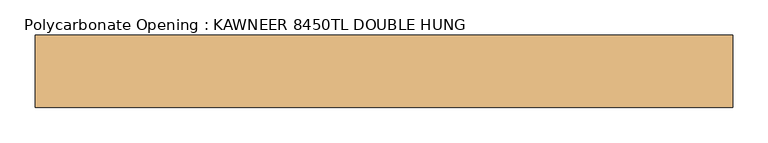
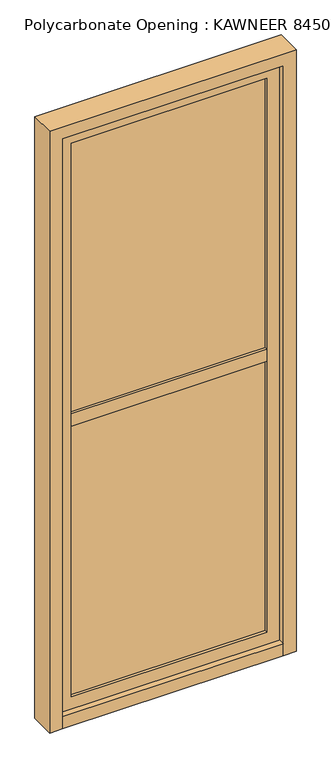
"""IFC4 building model written with IfcOpenShell, lengths in millimetres: door geometry, Polycarbonate Opening : KAWNEER 8450TL DOUBLE HUNG."""

from ifc_helpers import new_model, si_unit, frame, origin, origin_with_axes, place, context, project, spatial, polyline, outline, extrude, source, transform, mapped, element, save


def polycarbonate_opening_kawneer_8450tl_double_hung_37ce2fd3(model_context):
    return source(origin(), model_context, "Body", "SweptSolid", [
        extrude(outline(polyline([(440.1908884, 12.7), (440.1908884, -12.7), (-440.1908884, -12.7), (-440.1908884, 12.7), (440.1908884, 12.7)])), frame((0.0, 0.0, 50.8), z_axis=(0.0, 0.0, 1.0), x_axis=(1.0, 0.0, 0.0)), (0.0, 0.0, 1.0), 2434.1710618),
        extrude(outline(polyline([(2484.9710618, -440.1908884), (0.0, -440.1908884), (0.0, 440.1908884), (2484.9710618, 440.1908884), (2484.9710618, -440.1908884)]), holes=[polyline([(101.6, 389.3908884), (101.6, -389.3908884), (2434.1710618, -389.3908884), (2434.1710618, 389.3908884), (101.6, 389.3908884)])]), frame((0.0, -25.4, 0.0), z_axis=(0.0, 1.0, 0.0), x_axis=(0.0, 0.0, 1.0)), (0.0, 0.0, 1.0), 50.8),
        extrude(outline(polyline([(2535.7710618, 490.9908884), (2535.7710618, -490.9908884), (0.0, -490.9908884), (0.0, -440.1908884), (2484.9710618, -440.1908884), (2484.9710618, 440.1908884), (0.0, 440.1908884), (0.0, 490.9908884), (2535.7710618, 490.9908884)])), frame((0.0, -50.8, 0.0), z_axis=(0.0, 1.0, 0.0), x_axis=(0.0, 0.0, 1.0)), (0.0, 0.0, 1.0), 101.6),
        extrude(outline(polyline([(389.3908884, 25.4), (389.3908884, -25.4), (-389.3908884, -25.4), (-389.3908884, 25.4), (389.3908884, 25.4)])), frame((0.0, 0.0, 1242.4855309), z_axis=(0.0, 0.0, 1.0), x_axis=(1.0, 0.0, 0.0)), (0.0, 0.0, 1.0), 50.8),
        extrude(outline(polyline([(440.1908884, 50.8), (440.1908884, -50.8), (-440.1908884, -50.8), (-440.1908884, 50.8), (440.1908884, 50.8)])), origin_with_axes(), (0.0, 0.0, 1.0), 50.8),
    ])


if __name__ == "__main__":
    model = new_model("IFC4")
    model_context = context("Model", 3, world=origin())
    ifc_project = project(units=[si_unit("LENGTHUNIT", "METRE", prefix="MILLI")], contexts=[model_context])
    site = spatial("IfcSite", under=ifc_project)
    building = spatial("IfcBuilding", under=site)
    placement = place(None, origin())
    polycarbonate_opening_kawneer_8450tl_double_hung_shape = polycarbonate_opening_kawneer_8450tl_double_hung_37ce2fd3(model_context)
    element("IfcDoor", 1, ObjectType="Polycarbonate Opening : KAWNEER 8450TL DOUBLE HUNG", at=placement, inside=building, context=model_context, shape_type="MappedRepresentation", body=[
        mapped(polycarbonate_opening_kawneer_8450tl_double_hung_shape, transform((0.0, 0.0, 0.0), x_axis=(1.0, 0.0, 0.0), y_axis=(0.0, 1.0, 0.0), z_axis=(0.0, 0.0, 1.0))),
    ])
    save(model, "model.ifc")

# Revit data of these elements
# Type "Polycarbonate Opening : KAWNEER 8450TL DOUBLE HUNG"
#   Type Mark = "59"
#   OD_DS_Door_Material = "ALUM./GLAZING"
#   OD_DS_Door_Type = "STOREFRONT - DOUBLE HUNG WINDOW"
#   OD_DS_Lockset = "POLE OPERATOR HARDWARE FOR TOP SASH; BOTTOM SASH MECHANICALLY FIXED"
#   Analytic Construction = "<None>"
#   offset [instance default] = 0' - 2"
#   Stile = 0' - 2"
#   Mullion Width = 0' - 2"
#   Mullion Depth = 0' - 4"
#   Opening Size [instance default] = 5' - 1.50212"
#   Door Width [instance default] = 5' - 1.50212"
#   Window ON/OFF = no
#   Door On/Off = yes
#   Mullion Material = DOUBLE HUNG (CLEAR ANODIZED ALUM) - TEMPERED INSULATED GLAZING (CARDINAL GLASS LoĒ²-240\nOR EQUIVALENT)
#   Glass Material = TEMPERED INSULATED GLAZING (CARDINAL GLASS LoĒ²-240\nOR EQUIVALENT)
#   Door Material = DOUBLE HUNG (CLEAR ANODIZED ALUM) - TEMPERED INSULATED GLAZING (CARDINAL GLASS LoĒ²-240\nOR EQUIVALENT)
# Element 1 (IfcDoor, "Polycarbonate Opening : KAWNEER 8450TL DOUBLE HUNG")
#   offset = 0' - 0"
#   Materials on its faces: "DOUBLE HUNG (CLEAR ANODIZED ALUM) - TEMPERED INSULATED GLAZING (CARDINAL GLASS LoĒ²-240\nOR EQUIVALENT)", "TEMPERED INSULATED GLAZING (CARDINAL GLASS LoĒ²-240\nOR EQUIVALENT)"
# Materials
#   "DOUBLE HUNG (CLEAR ANODIZED ALUM) - TEMPERED INSULATED GLAZING (CARDINAL GLASS LoĒ²-240\nOR EQUIVALENT)": class "Metal", colour RGB 244 244 244, transparency 0, Description = "Aluminum 6061", Cost = 0
#   "TEMPERED INSULATED GLAZING (CARDINAL GLASS LoĒ²-240\nOR EQUIVALENT)": class "Glass", colour RGB 196 205 210, transparency 0.85, Description = "Soda Lime Glass", Cost = 0
